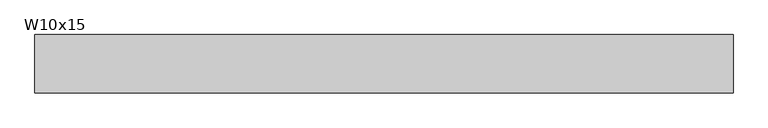
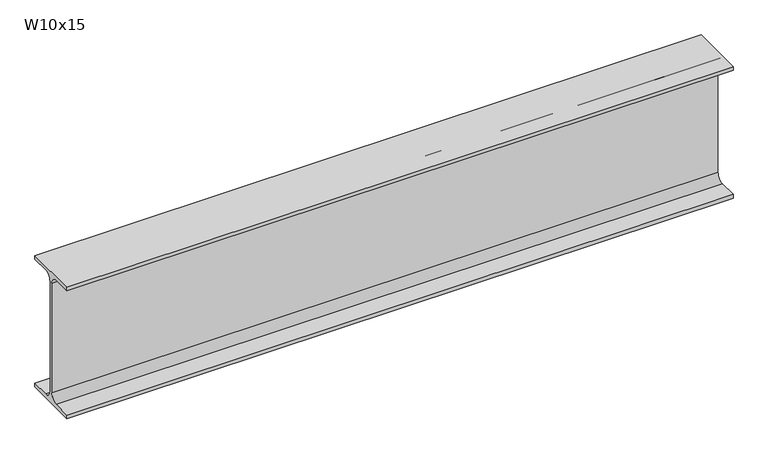
"""IFC4 building model written with IfcOpenShell, lengths in millimetres: beam geometry, RME W-Wide Flange : W10x15."""

from ifc_helpers import new_model, si_unit, point, frame, frame_2d, origin, place, context, project, spatial, polyline, circle_curve, trimmed, segment, composite_curve, outline, extrude, source, transform, mapped, element, save


def w10x15_31eddb5e(model_context):
    return source(origin(), model_context, "Body", "SweptSolid", [
        extrude(outline(composite_curve([segment(polyline([(50.8, -120.142), (50.8, -127.0), (-50.8, -127.0), (-50.8, -120.142), (-16.7005, -120.142)]), True, "CONTINUOUS"), segment(trimmed(circle_curve(frame_2d((-16.7005, -106.3625)), 13.7795), [point((-16.7005, -120.142))], [point((-2.921, -106.3625))], True, "CARTESIAN"), True, "CONTINUOUS"), segment(polyline([(-2.921, -106.3625), (-2.921, 106.3625)]), True, "CONTINUOUS"), segment(trimmed(circle_curve(frame_2d((-16.7005, 106.3625)), 13.7795), [point((-2.921, 106.3625))], [point((-16.7005, 120.142))], True, "CARTESIAN"), True, "CONTINUOUS"), segment(polyline([(-16.7005, 120.142), (-50.8, 120.142), (-50.8, 127.0), (50.8, 127.0), (50.8, 120.142), (16.7005, 120.142)]), True, "CONTINUOUS"), segment(trimmed(circle_curve(frame_2d((16.7005, 106.3625)), 13.7795), [point((16.7005, 120.142))], [point((2.921, 106.3625))], True, "CARTESIAN"), True, "CONTINUOUS"), segment(polyline([(2.921, 106.3625), (2.921, -106.3625)]), True, "CONTINUOUS"), segment(trimmed(circle_curve(frame_2d((16.7005, -106.3625)), 13.7795), [point((2.921, -106.3625))], [point((16.7005, -120.142))], True, "CARTESIAN"), True, "CONTINUOUS"), segment(polyline([(16.7005, -120.142), (50.8, -120.142)]), True, "CONTINUOUS")], self_intersect=False)), frame((-558.673, 0.0, 0.0), z_axis=(1.0, 0.0, 0.0), x_axis=(0.0, 1.0, 0.0)), (0.0, 0.0, 1.0), 1219.073),
    ])


if __name__ == "__main__":
    model = new_model("IFC4")
    model_context = context("Model", 3, world=origin())
    ifc_project = project(units=[si_unit("LENGTHUNIT", "METRE", prefix="MILLI")], contexts=[model_context])
    site = spatial("IfcSite", under=ifc_project)
    building = spatial("IfcBuilding", under=site)
    placement = place(None, origin())
    w10x15_shape = w10x15_31eddb5e(model_context)
    element("IfcBeam", 1, ObjectType="RME W-Wide Flange : W10x15", at=placement, inside=building, context=model_context, shape_type="MappedRepresentation", body=[
        mapped(w10x15_shape, transform((0.0, 0.0, 0.0), x_axis=(1.0, 0.0, 0.0), y_axis=(0.0, 1.0, 0.0), z_axis=(0.0, 0.0, 1.0))),
    ])
    save(model, "model.ifc")

# Revit data of these elements
# Type "RME W-Wide Flange : W10x15"
#   WELD P [instance default] = ""
#   WELD LE [instance default] = ""
#   WELD D [instance default] = ""
#   TOP SECTION SIZE [instance default] = ""
#   TOP SECTION LENGTH [instance default] = ""
#   REMARKS [instance default] = ""
#   REINF TYPE [instance default] = ""
#   Nominal Size = "W24"
#   End Bearing Capacity [instance default] = ""
#   BOT SECTION SIZE [instance default] = ""
#   BOT SECTION LENGTH [instance default] = ""
#   Assembly Code = "B10"
#   W = 15
#   Start Extension Calculation [instance default] = 10' - 0"
#   Start Extension [instance default] = -0' - 0 1/2"
#   End Extension Calculation [instance default] = 10' - 0"
#   End Extension [instance default] = -0' - 0 1/2"
#   Length [instance default] = 5' - 0"
#   bf = 0' - 4"
#   d = 0' - 10"
#   k = 0' - 0 13/16"
#   k2 = 0' - 0.5425"
#   tf = 0' - 0.27"
#   tw = 0' - 0.23"
#   A = 0.030625 SF
#   Structural Material [instance default] = Metal - Steel - ASTM A992
# Element 1 (IfcBeam, "RME W-Wide Flange : W10x15")
#   Length = 4' - 4"
#   Materials on its faces: "Metal - Steel - ASTM A992"
# Materials
#   "Metal - Steel - ASTM A992": class "Metal", colour RGB 255 128 0, transparency 0
